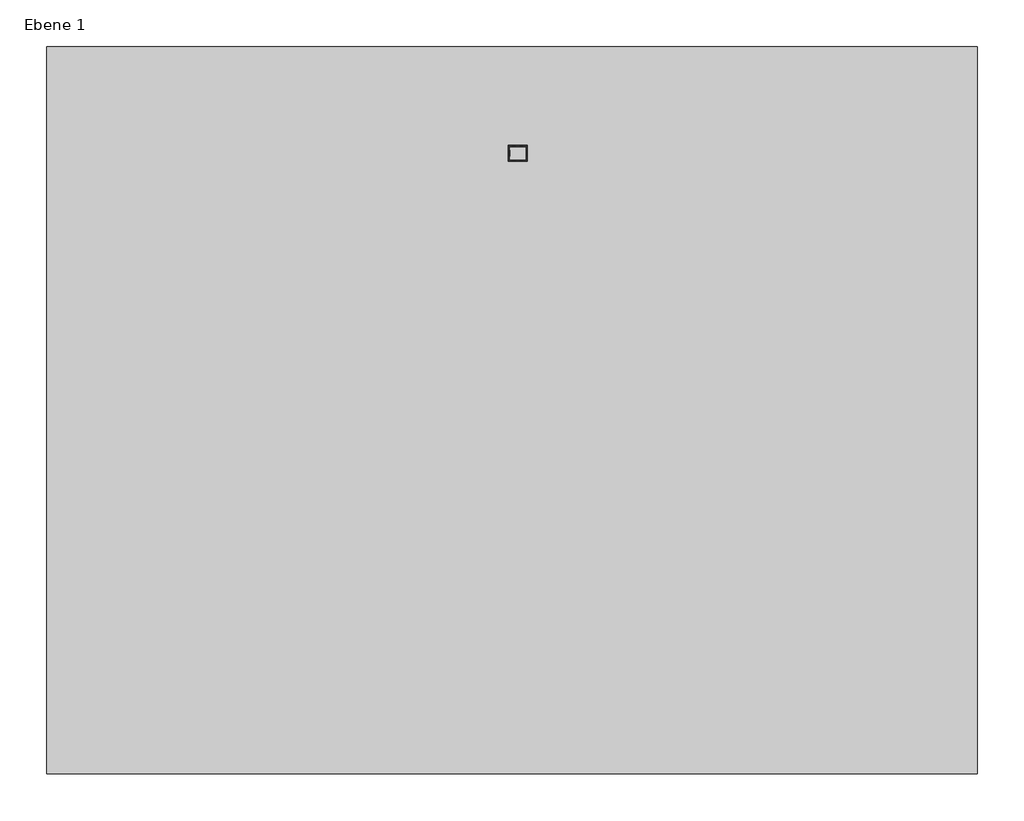
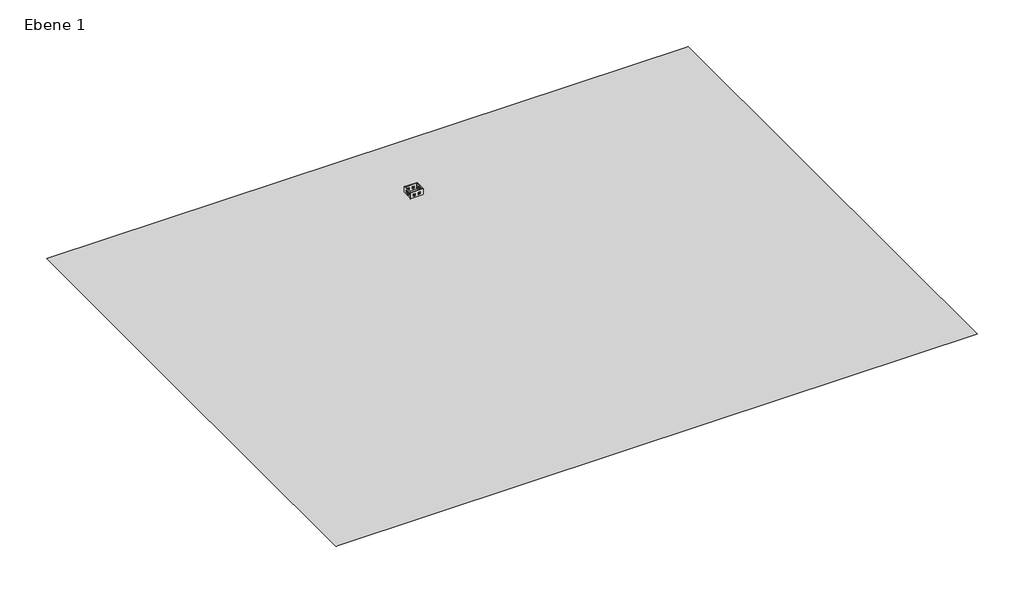
# One storey: 6 windows, 4 walls, 2 proxies.
"""IFC4 building model written with IfcOpenShell, lengths in millimetres."""

import ifcopenshell
import ifcopenshell.guid

model = None  # the IFC model being written
_history = None  # IfcOwnerHistory: only IFC2X3 demands one
_inside = {}  # id of a spatial element -> (the spatial element, [elements in it])
_under = {}  # id of a project, library or spatial element -> (it, [spatial elements below it])
_declared = {}  # id of a project -> (the project, [libraries it declares])
_typed = {}  # id of a type object -> (the type object, [elements of that type])
_made_of = {}  # id of a material, layer set ... -> (it, [elements and type objects made of it])


def new_model(schema):
    """Start an empty IFC model of exactly this schema.

    Asked for "IFC4X3", IfcOpenShell would pick the latest addendum, in which some entities
    have other attributes; the version numbers below select the first issue.
    IFC2X3 requires an IfcOwnerHistory on every rooted entity: one is made here for all.
    """
    global model, _history
    if schema == "IFC4X3":
        model = ifcopenshell.file(schema_version=(4, 3, 0, 0))
    else:
        model = ifcopenshell.file(schema=schema)
    _inside.clear()
    _under.clear()
    _declared.clear()
    _typed.clear()
    _made_of.clear()
    _history = None
    if model.schema == "IFC2X3":
        org = make("IfcOrganization", Name="unknown")
        user = make(
            "IfcPersonAndOrganization",
            ThePerson=make("IfcPerson", FamilyName="unknown"),
            TheOrganization=org,
        )
        app = make(
            "IfcApplication",
            ApplicationDeveloper=org,
            Version="unknown",
            ApplicationFullName="unknown",
            ApplicationIdentifier="unknown",
        )
        _history = make(
            "IfcOwnerHistory",
            OwningUser=user,
            OwningApplication=app,
            ChangeAction="ADDED",
            CreationDate=0,
        )
    return model


def make(cls, **values):
    """One entity of the class cls with the attributes given. An attribute that is None is left unset."""
    return model.create_entity(
        cls, **{name: value for name, value in values.items() if value is not None}
    )


def rooted(cls, **values):
    """An entity with a GlobalId (a new one), such as an element, a storey or a relation."""
    return make(cls, GlobalId=ifcopenshell.guid.new(), OwnerHistory=_history, **values)


def si_unit(unit_type, name, prefix=None):
    """IfcSIUnit, for example si_unit("LENGTHUNIT", "METRE", prefix="MILLI")."""
    return make("IfcSIUnit", UnitType=unit_type, Prefix=prefix, Name=name)


def assignment(units):
    """IfcUnitAssignment: the units of a project."""
    return None if units is None else make("IfcUnitAssignment", Units=units)


def point(xyz):
    """IfcCartesianPoint."""
    return None if xyz is None else make("IfcCartesianPoint", Coordinates=xyz)


def direction(xyz):
    """IfcDirection."""
    return None if xyz is None else make("IfcDirection", DirectionRatios=xyz)


def frame(location, z_axis=None, x_axis=None):
    """IfcAxis2Placement3D, a coordinate frame: its origin and axes. An axis left out is left unset."""
    return make(
        "IfcAxis2Placement3D",
        Location=point(location),
        Axis=direction(z_axis),
        RefDirection=direction(x_axis),
    )


def origin():
    """The frame at (0, 0, 0) with its axes left unset."""
    return frame((0.0, 0.0, 0.0))


def place(relative_to, where):
    """IfcLocalPlacement: puts the frame where relative to a parent placement (None: the world)."""
    return make(
        "IfcLocalPlacement", PlacementRelTo=relative_to, RelativePlacement=where
    )


def context(
    kind, dimensions, precision=None, world=None, true_north=None, identifier=None
):
    """IfcGeometricRepresentationContext, for example the 3D "Model" context."""
    return make(
        "IfcGeometricRepresentationContext",
        ContextIdentifier=identifier,
        ContextType=kind,
        CoordinateSpaceDimension=dimensions,
        Precision=precision,
        WorldCoordinateSystem=world,
        TrueNorth=true_north,
    )


def project(units=None, contexts=None):
    """IfcProject with its units and contexts."""
    return rooted(
        "IfcProject",
        Name="project",
        RepresentationContexts=contexts,
        UnitsInContext=assignment(units),
    )


def spatial(cls, under=None, at=None, **own):
    """A site, building, storey or space (cls), placed at a placement, below another one or the project."""
    s = rooted(cls, ObjectPlacement=at, **own)
    if under is not None:
        _under.setdefault(under.id(), (under, []))[1].append(s)
    return s


def polyline(points):
    """IfcPolyline through the points."""
    return make("IfcPolyline", Points=[point(p) for p in points])


def point_list(points):
    """IfcCartesianPointList2D or 3D."""
    cls = (
        "IfcCartesianPointList2D" if len(points[0]) == 2 else "IfcCartesianPointList3D"
    )
    return make(cls, CoordList=points)


def outline(outer, holes=None, kind="AREA"):
    """IfcArbitraryClosedProfileDef: a profile drawn as a closed curve; with holes, ...WithVoids."""
    if holes is None:
        return make("IfcArbitraryClosedProfileDef", ProfileType=kind, OuterCurve=outer)
    return make(
        "IfcArbitraryProfileDefWithVoids",
        ProfileType=kind,
        OuterCurve=outer,
        InnerCurves=holes,
    )


def extrude(swept, where, along, depth):
    """IfcExtrudedAreaSolid: the profile swept, set in the frame where, extruded along a direction by depth."""
    return make(
        "IfcExtrudedAreaSolid",
        SweptArea=swept,
        Position=where,
        ExtrudedDirection=direction(along),
        Depth=depth,
    )


def faces_of(points, faces, orient=None, outer=None):
    """IfcFace entities. A face is a list of loops; a loop is a list of indices into points, from 0.

    orient and outer hold one flag for each loop. By default every Orientation is true, the
    first loop of a face is its IfcFaceOuterBound and the others are IfcFaceBound.
    """
    made = []
    for i, loops in enumerate(faces):
        bounds = []
        for j, loop in enumerate(loops):
            is_outer = j == 0 if outer is None else outer[i][j]
            bounds.append(
                make(
                    "IfcFaceOuterBound" if is_outer else "IfcFaceBound",
                    Bound=make("IfcPolyLoop", Polygon=[points[k] for k in loop]),
                    Orientation=True if orient is None else orient[i][j],
                )
            )
        made.append(make("IfcFace", Bounds=bounds))
    return made


def faceted_brep(points, faces, orient=None, outer=None, voids=None):
    """IfcFacetedBrep: a solid bounded by flat faces; with voids (closed shells), ...WithVoids."""
    shared = [point(p) for p in points]
    hull = make("IfcClosedShell", CfsFaces=faces_of(shared, faces, orient, outer))
    if voids is None:
        return make("IfcFacetedBrep", Outer=hull)
    return make(
        "IfcFacetedBrepWithVoids",
        Outer=hull,
        Voids=[
            make(cls, CfsFaces=faces_of(shared, fs, o, b)) for cls, fs, o, b in voids
        ],
    )


def triangles(points, corners, closed=None, point_numbers=None):
    """IfcTriangulatedFaceSet: each triangle names its three corners, points numbered from 1."""
    return make(
        "IfcTriangulatedFaceSet",
        Coordinates=point_list(points),
        Closed=closed,
        CoordIndex=corners,
        PnIndex=point_numbers,
    )


def shape(context_of_items, identifier, shape_type, items):
    """IfcShapeRepresentation: the items that make up one representation, for example the "Body"."""
    return make(
        "IfcShapeRepresentation",
        ContextOfItems=context_of_items,
        RepresentationIdentifier=identifier,
        RepresentationType=shape_type,
        Items=items,
    )


def source(mapping_origin, context_of_items, identifier, shape_type, items):
    """IfcRepresentationMap: a shape defined once, which mapped items show again and again."""
    return make(
        "IfcRepresentationMap",
        MappingOrigin=mapping_origin,
        MappedRepresentation=shape(context_of_items, identifier, shape_type, items),
    )


def transform(
    local_origin,
    x_axis=None,
    y_axis=None,
    z_axis=None,
    scale=None,
    scale2=None,
    scale3=None,
    uniform=True,
):
    """IfcCartesianTransformationOperator3D, or its non-uniform kind. x_axis, y_axis, z_axis: its Axis1, 2, 3."""
    if uniform:
        return make(
            "IfcCartesianTransformationOperator3D",
            Axis1=direction(x_axis),
            Axis2=direction(y_axis),
            LocalOrigin=point(local_origin),
            Scale=scale,
            Axis3=direction(z_axis),
        )
    return make(
        "IfcCartesianTransformationOperator3DnonUniform",
        Axis1=direction(x_axis),
        Axis2=direction(y_axis),
        LocalOrigin=point(local_origin),
        Scale=scale,
        Axis3=direction(z_axis),
        Scale2=scale2,
        Scale3=scale3,
    )


def mapped(mapping_source, mapping_target):
    """IfcMappedItem: shows the shape of a source again, moved by a transform."""
    return make(
        "IfcMappedItem", MappingSource=mapping_source, MappingTarget=mapping_target
    )


def made_of(thing, what):
    """Note that an element or type object is made of a material, layer set ...; save() writes the relation."""
    if what is not None:
        _made_of.setdefault(what.id(), (what, []))[1].append(thing)
    return thing


def element(
    cls,
    number,
    at=None,
    inside=None,
    cuts=None,
    type_object=None,
    material=None,
    context=None,
    identifier="Body",
    shape_type=None,
    held_by="IfcProductDefinitionShape",
    body=None,
    shapes=None,
    **own,
):
    """One element of the class cls, such as IfcWall. Its Tag is "e" and its number.

    at: its placement. inside: the storey or other place that contains it. cuts: it is an
    opening in that element (IfcRelVoidsElement). A single representation is given by context,
    identifier, shape_type and body (its items); several are given by shapes. held_by: the class
    of the entity that holds the representations. save() writes the other relations.
    """
    e = rooted(cls, Tag="e%d" % number, ObjectPlacement=at, **own)
    if body is not None:
        shapes = [shape(context, identifier, shape_type, body)]
    if shapes is not None:
        e.Representation = make(held_by, Representations=shapes)
    if inside is not None:
        _inside.setdefault(inside.id(), (inside, []))[1].append(e)
    if cuts is not None:
        rooted(
            "IfcRelVoidsElement", RelatingBuildingElement=cuts, RelatedOpeningElement=e
        )
    if type_object is not None:
        _typed.setdefault(type_object.id(), (type_object, []))[1].append(e)
    return made_of(e, material)


def aggregate(whole, parts):
    """IfcRelAggregates: a whole, such as a stair, and the parts it consists of."""
    return rooted("IfcRelAggregates", RelatingObject=whole, RelatedObjects=parts)


def save(model, path):
    """Write the relations noted so far, then the file.

    IfcRelAggregates (storeys below a building ...), IfcRelContainedInSpatialStructure (elements
    in a storey), IfcRelDefinesByType, IfcRelAssociatesMaterial and IfcRelDeclares: one each for
    every whole, place, type object, material and project.
    """
    for whole, parts in _under.values():
        aggregate(whole, parts)
    for where, things in _inside.values():
        rooted(
            "IfcRelContainedInSpatialStructure",
            RelatedElements=things,
            RelatingStructure=where,
        )
    for kind, things in _typed.values():
        rooted("IfcRelDefinesByType", RelatedObjects=things, RelatingType=kind)
    for what, things in _made_of.values():
        rooted("IfcRelAssociatesMaterial", RelatedObjects=things, RelatingMaterial=what)
    for by, libraries in _declared.values():
        rooted("IfcRelDeclares", RelatingContext=by, RelatedDefinitions=libraries)
    model.write(path)


def fenster_1_flg_variabel_fenster_1_flg_variabel_3_8a378bad(model_context):
    return source(origin(), model_context, "Body", "SolidModel", [
        extrude(outline(polyline([(2010.0, 505.0), (2010.0, -505.0), (1000.0, -505.0), (1000.0, 505.0), (2010.0, 505.0)]), holes=[polyline([(1930.0, 445.0), (1080.0, 445.0), (1080.0, -445.0), (1930.0, -445.0), (1930.0, 445.0)])]), frame((0.0, 40.0, 0.0), z_axis=(0.0, 1.0, 0.0), x_axis=(0.0, 0.0, 1.0)), (0.0, 0.0, 1.0), 60.0),
        faceted_brep([(475.0, 40.0, 1960.0), (475.0, 10.0, 1960.0), (475.0, 10.0, 1050.0), (475.0, 40.0, 1050.0), (-475.0, 10.0, 1960.0), (-475.0, 10.0, 1050.0), (415.0, 10.0, 1110.0), (-415.0, 10.0, 1110.0), (-415.0, 10.0, 1900.0), (415.0, 10.0, 1900.0), (-475.0, 40.0, 1050.0), (-475.0, 40.0, 1960.0), (445.0, 40.0, 1930.0), (-445.0, 40.0, 1930.0), (-445.0, 40.0, 1080.0), (445.0, 40.0, 1080.0), (445.0, 70.0, 1930.0), (445.0, 70.0, 1080.0), (-445.0, 70.0, 1080.0), (-445.0, 70.0, 1930.0), (415.0, 70.0, 1900.0), (-415.0, 70.0, 1900.0), (-415.0, 70.0, 1110.0), (415.0, 70.0, 1110.0)], [[[0, 1, 2, 3]], [[1, 4, 5, 2], [6, 7, 8, 9]], [[3, 2, 5, 10]], [[3, 10, 11, 0], [12, 13, 14, 15]], [[16, 12, 15, 17]], [[17, 15, 14, 18]], [[17, 18, 19, 16], [20, 21, 22, 23]], [[9, 20, 23, 6]], [[6, 23, 22, 7]], [[10, 5, 4, 11]], [[18, 14, 13, 19]], [[7, 22, 21, 8]], [[11, 4, 1, 0]], [[19, 13, 12, 16]], [[8, 21, 20, 9]]]),
        extrude(outline(polyline([(-505.0, -210.0), (-505.0, 40.0), (505.0, 40.0), (505.0, -210.0), (-505.0, -210.0)])), frame((0.0, 0.0, 1005.0), z_axis=(0.0, 0.0, 1.0), x_axis=(1.0, 0.0, 0.0)), (0.0, 0.0, 1.0), 15.0),
        extrude(outline(polyline([(110.0221543, 1020.0), (210.0, 1000.0), (210.0, 990.0), (208.0, 990.0), (208.0, 998.3604634), (109.8240723, 1018.0), (100.0, 1018.0), (100.0, 1020.0), (110.0221543, 1020.0)])), frame((-505.0, 0.0, 0.0), z_axis=(1.0, 0.0, 0.0), x_axis=(0.0, 1.0, 0.0)), (0.0, 0.0, 1.0), 1010.0),
        extrude(outline(polyline([(415.0, 25.0), (-415.0, 25.0), (-415.0, 55.0), (415.0, 55.0), (415.0, 25.0)])), frame((0.0, 0.0, 1110.0), z_axis=(0.0, 0.0, 1.0), x_axis=(1.0, 0.0, 0.0)), (0.0, 0.0, 1.0), 790.0),
    ])


def fenster_2_flg_variabel_fenster_2_flg_variabel_3_03287464(model_context):
    return source(origin(), model_context, "Body", "SolidModel", [
        extrude(outline(polyline([(60.0, -5.0), (915.0, -5.0), (915.0, -35.0), (60.0, -35.0), (60.0, -5.0)])), frame((0.0, 0.0, 1110.0), z_axis=(0.0, 0.0, 1.0), x_axis=(1.0, 0.0, 0.0)), (0.0, 0.0, 1.0), 1040.0),
        extrude(outline(polyline([(-915.0, -5.0), (-60.0, -5.0), (-60.0, -35.0), (-915.0, -35.0), (-915.0, -5.0)])), frame((0.0, 0.0, 1110.0), z_axis=(0.0, 0.0, 1.0), x_axis=(1.0, 0.0, 0.0)), (0.0, 0.0, 1.0), 1040.0),
        extrude(outline(polyline([(-1005.0, -210.0), (-1005.0, -20.0), (1005.0, -20.0), (1005.0, -210.0), (-1005.0, -210.0)])), frame((0.0, 0.0, 1005.0), z_axis=(0.0, 0.0, 1.0), x_axis=(1.0, 0.0, 0.0)), (0.0, 0.0, 1.0), 15.0),
        extrude(outline(polyline([(50.0221543, 1020.0), (210.0, 1000.0), (210.0, 990.0), (208.0, 990.0), (208.0, 998.3604634), (49.8240723, 1018.0), (40.0, 1018.0), (40.0, 1020.0), (50.0221543, 1020.0)])), frame((-1005.0, 0.0, 0.0), z_axis=(1.0, 0.0, 0.0), x_axis=(0.0, 1.0, 0.0)), (0.0, 0.0, 1.0), 2010.0),
        extrude(outline(polyline([(30.0, -20.0), (-30.0, -20.0), (-30.0, 40.0), (30.0, 40.0), (30.0, -20.0)])), frame((0.0, 0.0, 1080.0), z_axis=(0.0, 0.0, 1.0), x_axis=(1.0, 0.0, 0.0)), (0.0, 0.0, 1.0), 1100.0),
        extrude(outline(polyline([(2260.0, -1005.0), (1000.0, -1005.0), (1000.0, 1005.0), (2260.0, 1005.0), (2260.0, -1005.0)]), holes=[polyline([(2180.0, -945.0), (2180.0, 945.0), (1080.0, 945.0), (1080.0, -945.0), (2180.0, -945.0)])]), frame((0.0, -20.0, 0.0), z_axis=(0.0, 1.0, 0.0), x_axis=(0.0, 0.0, 1.0)), (0.0, 0.0, 1.0), 60.0),
        faceted_brep([(-945.0, -20.0, 1080.0), (-945.0, 10.0, 1080.0), (-30.0, 10.0, 1080.0), (-30.0, -20.0, 1080.0), (-30.0, 10.0, 2180.0), (-30.0, -20.0, 2180.0), (-945.0, 10.0, 2180.0), (-60.0, 10.0, 2150.0), (-915.0, 10.0, 2150.0), (-915.0, 10.0, 1110.0), (-60.0, 10.0, 1110.0), (0.0, -20.0, 1050.0), (-975.0, -20.0, 1050.0), (-975.0, -20.0, 2210.0), (0.0, -20.0, 2210.0), (-945.0, -20.0, 2180.0), (-975.0, -50.0, 1050.0), (0.0, -50.0, 1050.0), (0.0, -50.0, 2210.0), (-975.0, -50.0, 2210.0), (-60.0, -50.0, 1110.0), (-915.0, -50.0, 1110.0), (-915.0, -50.0, 2150.0), (-60.0, -50.0, 2150.0)], [[[0, 1, 2, 3]], [[3, 2, 4, 5]], [[2, 1, 6, 4], [7, 8, 9, 10]], [[11, 12, 13, 14], [5, 15, 0, 3]], [[16, 12, 11, 17]], [[17, 11, 14, 18]], [[18, 19, 16, 17], [20, 21, 22, 23]], [[9, 21, 20, 10]], [[10, 20, 23, 7]], [[15, 6, 1, 0]], [[19, 13, 12, 16]], [[8, 22, 21, 9]], [[5, 4, 6, 15]], [[18, 14, 13, 19]], [[7, 23, 22, 8]]]),
        faceted_brep([(30.0, -20.0, 1080.0), (30.0, 10.0, 1080.0), (945.0, 10.0, 1080.0), (945.0, -20.0, 1080.0), (945.0, 10.0, 2180.0), (945.0, -20.0, 2180.0), (30.0, 10.0, 2180.0), (915.0, 10.0, 2150.0), (60.0, 10.0, 2150.0), (60.0, 10.0, 1110.0), (915.0, 10.0, 1110.0), (975.0, -20.0, 1050.0), (0.0, -20.0, 1050.0), (0.0, -20.0, 2210.0), (975.0, -20.0, 2210.0), (30.0, -20.0, 2180.0), (0.0, -50.0, 1050.0), (975.0, -50.0, 1050.0), (975.0, -50.0, 2210.0), (0.0, -50.0, 2210.0), (915.0, -50.0, 1110.0), (60.0, -50.0, 1110.0), (60.0, -50.0, 2150.0), (915.0, -50.0, 2150.0)], [[[0, 1, 2, 3]], [[3, 2, 4, 5]], [[2, 1, 6, 4], [7, 8, 9, 10]], [[11, 12, 13, 14], [5, 15, 0, 3]], [[16, 12, 11, 17]], [[17, 11, 14, 18]], [[18, 19, 16, 17], [20, 21, 22, 23]], [[9, 21, 20, 10]], [[10, 20, 23, 7]], [[15, 6, 1, 0]], [[19, 13, 12, 16]], [[8, 22, 21, 9]], [[5, 4, 6, 15]], [[18, 14, 13, 19]], [[7, 23, 22, 8]]]),
    ])


model = new_model("IFC4")

# Units and contexts
model_context = context("Model", 3, world=origin())
ifc_project = project(units=[si_unit("LENGTHUNIT", "METRE", prefix="MILLI")], contexts=[model_context])

# Site, building, storey
site = spatial("IfcSite", under=ifc_project)
building = spatial("IfcBuilding", under=site)
storey = spatial("IfcBuildingStorey", under=building, Name="Ebene 1", Elevation=3000.0)

# Proxies
placement = place(None, origin())
element("IfcBuildingElementProxy", 1, Name="Building Element Proxy", at=placement, inside=storey, context=model_context, shape_type="Tessellation", body=[
    triangles([(-160331.1996094, -65742.4011108, 3048.0), (-160331.1996094, -208151.4062988, 3048.0), (23848.9001038, -208151.4062988, 3048.0), (12197.4996643, -199419.9020508, 3048.0), (-5694.3001007, -186011.6041992, 3048.0), (-25481.9004272, -171004.4085938, 3048.0), (-41498.6018555, -156049.302832, 3048.0), (-55953.3009521, -142550.7035156, 3048.0), (-81517.601001, -122551.5986572, 3048.0), (-90344.9970703, -115644.9969727, 3048.0), (-95745.3, -111898.3977539, 3048.0), (-139582.1033203, -81515.7034424, 3048.0), (154493.6024414, -208151.4062988, 3048.0), (154493.6024414, -146509.2990967, 3048.0), (152327.2974609, -183778.6986328, 3048.0), (151970.2029785, -191029.9025391, 3048.0), (131234.6407471, -189976.3854492, 3048.0), (128010.9956543, -189812.6000977, 3048.0), (103567.5016113, -191451.7000488, 3048.0), (73532.4977051, -193637.296875, 3048.0), (59545.7979492, -197106.1083984, 3048.0), (45621.6990234, -200561.3021484, 3048.0), (35421.8006836, -204117.6060059, 3048.0), (25840.2994812, -207458.2951172, 3048.0), (154493.6024414, 37859.0007568, 3048.0), (-45179.0004639, 37859.0007568, 3048.0), (-20995.999823, -3482.9999016, 3048.0), (-20185.0004883, -4870.0001244, 3048.0), (-16502.099707, -11166.2998169, 3048.0), (-5863.3002502, -5298.2998535, 3048.0), (4055.6001251, 223.0999905, 3048.0), (14232.299881, 5042.7997513, 3048.0), (20896.8988953, 7816.7002029, 3048.0), (23379.4008545, 2726.9001228, 3048.0), (32183.900647, -15324.6994812, 3048.0), (35127.4000488, -15951.6995819, 3048.0), (51396.7000122, -19416.9996918, 3048.0), (71552.5022827, -34777.0005066, 3048.0), (89162.3994873, -48196.3000122, 3048.0), (97424.6021484, -54516.300293, 3048.0), (103453.3969482, -59668.902063, 3048.0), (125381.6956787, -79503.9006592, 3048.0), (138980.4005127, -76672.5013916, 3048.0), (142103.1959473, -85544.0994141, 3048.0), (152666.9046387, -116932.3044434, 3048.0), (-160331.1996094, 37859.0007568, 3048.0), (-157617.8024414, -59206.6000488, 3048.0), (-156348.2055176, -56148.4006714, 3048.0), (-133528.5007324, -3798.9000961, 3048.0), (-116015.0022949, -11087.9999451, 3048.0), (-107594.0000244, -6686.0000336, 3048.0), (-104346.1517578, -5888.8399704, 3048.0), (-103918.9964355, -5783.9998581, 3048.0), (-102571.999585, -5452.9997131, 3048.0), (-102346.0040771, -5318.9997528, 3048.0), (-100888.0000488, -4452.9999962, 3048.0), (-98390.0036865, -3171.9999893, 3048.0), (-95145.0017578, -1507.0000202, 3048.0), (-87760.0013672, 3877.9999191, 3048.0), (-87175.9998047, 4304.0000793, 3048.0), (-73718.9979492, 7734.0000183, 3048.0), (-75124.0005615, 10122.9995453, 3048.0), (-76451.9985718, 12378.0002747, 3048.0), (-73623.9990967, 14575.9998322, 3048.0), (-67567.0013672, 20473.9991272, 3048.0), (-64063.0012939, 24429.9995178, 3048.0), (-58507.0008911, 30701.0004639, 3048.0), (-58376.9995239, 30747.9999207, 3048.0)], [[1, 2, 12], [47, 12, 48], [12, 47, 1], [50, 12, 11], [46, 1, 47], [48, 50, 49], [48, 12, 50], [56, 51, 52], [52, 51, 50], [50, 53, 52], [50, 51, 49], [12, 2, 11], [46, 47, 48], [10, 29, 11], [9, 2, 8], [9, 29, 10], [8, 2, 7], [10, 2, 9], [9, 8, 29], [53, 54, 55], [53, 50, 54], [57, 55, 11], [11, 55, 54], [11, 2, 10], [58, 11, 29], [50, 11, 54], [52, 53, 56], [35, 8, 7], [7, 2, 6], [2, 5, 6], [55, 56, 53], [51, 57, 49], [57, 51, 56], [49, 57, 59], [57, 11, 58], [55, 57, 56], [59, 57, 58], [46, 59, 60], [59, 46, 49], [60, 63, 46], [63, 60, 62], [59, 61, 60], [46, 63, 65], [58, 61, 59], [49, 46, 48], [62, 61, 64], [61, 62, 60], [65, 61, 27], [61, 65, 64], [27, 61, 28], [62, 64, 63], [66, 46, 65], [65, 27, 66], [67, 68, 26], [68, 67, 66], [68, 66, 27], [67, 26, 46], [26, 68, 27], [67, 46, 66], [27, 31, 26], [63, 64, 65], [58, 29, 61], [7, 6, 38], [4, 3, 24], [24, 13, 23], [4, 24, 23], [21, 22, 23], [21, 23, 13], [4, 23, 22], [4, 22, 5], [4, 5, 2], [5, 21, 39], [13, 20, 21], [22, 21, 5], [20, 40, 21], [24, 3, 13], [3, 4, 2], [18, 13, 17], [13, 18, 19], [16, 13, 15], [13, 16, 17], [19, 20, 13], [17, 16, 15], [19, 18, 14], [42, 19, 45], [45, 19, 14], [14, 15, 13], [45, 14, 25], [18, 17, 14], [17, 15, 14], [44, 45, 25], [19, 42, 20], [44, 42, 45], [28, 29, 30], [28, 61, 29], [30, 35, 31], [35, 30, 29], [35, 29, 8], [30, 31, 27], [32, 26, 31], [32, 31, 34], [37, 33, 34], [34, 33, 32], [31, 35, 34], [33, 26, 32], [34, 35, 36], [28, 30, 27], [25, 40, 41], [39, 38, 6], [42, 43, 41], [43, 42, 44], [40, 39, 21], [25, 41, 43], [37, 25, 33], [37, 36, 38], [38, 39, 25], [36, 35, 7], [25, 39, 40], [38, 25, 37], [38, 36, 7], [37, 34, 36], [43, 44, 25], [41, 40, 20], [20, 42, 41], [33, 25, 26], [39, 6, 5]], closed=False),
])
element("IfcBuildingElementProxy", 2, Name="Building Element Proxy", at=placement, inside=storey, context=model_context, shape_type="Tessellation", body=[
    triangles([(-20995.999823, -3482.9999016, 3048.0), (-45179.0004639, 37859.0007568, 3048.0), (-58376.9995239, 30747.9999207, 3048.0), (-58507.0008911, 30701.0004639, 3048.0), (-64063.0012939, 24429.9995178, 3048.0), (-67567.0013672, 20473.9991272, 3048.0), (-73623.9990967, 14575.9998322, 3048.0), (-76451.9985718, 12378.0002747, 3048.0), (-75124.0005615, 10122.9995453, 3048.0), (-73718.9979492, 7734.0000183, 3048.0), (-87175.9998047, 4304.0000793, 3048.0), (-87760.0013672, 3877.9999191, 3048.0), (-95145.0017578, -1507.0000202, 3048.0), (-98390.0036865, -3171.9999893, 3048.0), (-100888.0000488, -4452.9999962, 3048.0), (-102346.0040771, -5318.9997528, 3048.0), (-102571.999585, -5452.9997131, 3048.0), (-103918.9964355, -5783.9998581, 3048.0), (-104346.1517578, -5888.8399704, 3048.0), (-107594.0000244, -6686.0000336, 3048.0), (-116015.0022949, -11087.9999451, 3048.0), (-133528.5007324, -3798.9000961, 3048.0), (-156348.2055176, -56148.4006714, 3048.0), (-157617.8024414, -59206.6000488, 3048.0), (-160331.1996094, -65742.4011108, 3048.0), (-139582.1033203, -81515.7034424, 3048.0), (-95745.3, -111898.3977539, 3048.0), (-90344.9970703, -115644.9969727, 3048.0), (-81517.601001, -122551.5986572, 3048.0), (-55953.3009521, -142550.7035156, 3048.0), (-41498.6018555, -156049.302832, 3048.0), (-25481.9004272, -171004.4085938, 3048.0), (-5694.3001007, -186011.6041992, 3048.0), (12197.4996643, -199419.9020508, 3048.0), (23848.9001038, -208151.4062988, 3048.0), (25840.2994812, -207458.2951172, 3048.0), (35421.8006836, -204117.6060059, 3048.0), (45621.6990234, -200561.3021484, 3048.0), (59545.7979492, -197106.1083984, 3048.0), (73532.4977051, -193637.296875, 3048.0), (103567.5016113, -191451.7000488, 3048.0), (128010.9956543, -189812.6000977, 3048.0), (131234.6407471, -189976.3854492, 3048.0), (151970.2029785, -191029.9025391, 3048.0), (152327.2974609, -183778.6986328, 3048.0), (154493.6024414, -146509.2990967, 3048.0), (152666.9046387, -116932.3044434, 3048.0), (142103.1959473, -85544.0994141, 3048.0), (138980.4005127, -76672.5013916, 3048.0), (125381.6956787, -79503.9006592, 3048.0), (103453.3969482, -59668.902063, 3048.0), (97424.6021484, -54516.300293, 3048.0), (89162.3994873, -48196.3000122, 3048.0), (71552.5022827, -34777.0005066, 3048.0), (51396.7000122, -19416.9996918, 3048.0), (35127.4000488, -15951.6995819, 3048.0), (32183.900647, -15324.6994812, 3048.0), (23379.4008545, 2726.9001228, 3048.0), (20896.8988953, 7816.7002029, 3048.0), (14232.299881, 5042.7997513, 3048.0), (4055.6001251, 223.0999905, 3048.0), (-5863.3002502, -5298.2998535, 3048.0), (-16502.099707, -11166.2998169, 3048.0), (-20185.0004883, -4870.0001244, 3048.0)], [[24, 25, 26], [23, 26, 21], [26, 23, 24], [20, 21, 19], [18, 19, 21], [18, 21, 17], [21, 26, 27], [23, 21, 22], [28, 63, 27], [29, 63, 28], [29, 30, 63], [16, 17, 27], [16, 27, 14], [17, 21, 27], [13, 27, 63], [57, 30, 31], [14, 27, 13], [16, 14, 15], [8, 9, 7], [10, 11, 12], [12, 13, 10], [10, 7, 9], [7, 10, 6], [6, 1, 5], [1, 6, 10], [1, 10, 64], [4, 5, 3], [3, 5, 1], [1, 2, 3], [13, 63, 10], [31, 32, 54], [34, 35, 36], [34, 36, 37], [34, 37, 38], [34, 38, 33], [33, 39, 53], [38, 39, 33], [40, 52, 39], [41, 42, 46], [42, 43, 46], [45, 43, 44], [46, 47, 41], [46, 43, 45], [41, 47, 50], [41, 50, 40], [48, 50, 47], [64, 10, 63], [62, 57, 61], [57, 62, 63], [57, 63, 30], [60, 61, 58], [58, 59, 60], [61, 57, 58], [53, 54, 32], [49, 50, 48], [52, 53, 39], [55, 56, 54], [56, 57, 31], [54, 56, 31], [51, 52, 40], [40, 50, 51], [53, 32, 33]], closed=False),
])

# Walls
element("IfcWall", 3, ObjectType="MW 24.0 WD 12.0", at=placement, inside=storey, context=model_context, shape_type="Brep", body=[
    faceted_brep([(-3766.4979049, 4044.3692517, 3000.0), (1873.5020951, 4044.3692517, 3000.0), (1873.5020951, 4044.3692517, 6000.0), (-3766.4979049, 4044.3692517, 6000.0), (673.5020951, 4044.3692517, 4000.0), (-336.4979049, 4044.3692517, 4000.0), (-336.4979049, 4044.3692517, 5010.0), (673.5020951, 4044.3692517, 5010.0), (-1756.4979049, 4044.3692517, 4000.0), (-2766.4979049, 4044.3692517, 4000.0), (-2766.4979049, 4044.3692517, 5010.0), (-1756.4979049, 4044.3692517, 5010.0), (-4126.4979049, 4404.3692517, 3000.0), (-4126.4979049, 4404.3692517, 6000.0), (2233.5020951, 4404.3692517, 6000.0), (2233.5020951, 4404.3692517, 3000.0), (673.5020951, 4404.3692517, 4000.0), (673.5020951, 4404.3692517, 5010.0), (-336.4979049, 4404.3692517, 5010.0), (-336.4979049, 4404.3692517, 4000.0), (-1756.4979049, 4404.3692517, 4000.0), (-1756.4979049, 4404.3692517, 5010.0), (-2766.4979049, 4404.3692517, 5010.0), (-2766.4979049, 4404.3692517, 4000.0)], [[[0, 1, 2, 3], [4, 5, 6, 7], [8, 9, 10, 11]], [[12, 13, 14, 15], [16, 17, 18, 19], [20, 21, 22, 23]], [[1, 0, 12, 15]], [[3, 2, 14, 13]], [[2, 1, 15, 14]], [[0, 3, 13, 12]], [[17, 16, 4, 7]], [[18, 17, 7, 6]], [[19, 18, 6, 5]], [[16, 19, 5, 4]], [[21, 20, 8, 11]], [[22, 21, 11, 10]], [[23, 22, 10, 9]], [[20, 23, 9, 8]]]),
])
element("IfcWall", 4, ObjectType="MW 24.0 WD 12.0", at=placement, inside=storey, context=model_context, shape_type="Brep", body=[
    faceted_brep([(1873.5020951, 4044.3692517, 3000.0), (1873.5020951, -595.6307483, 3000.0), (1873.5020951, -595.6307483, 6000.0), (1873.5020951, 4044.3692517, 6000.0), (1873.5020951, 719.3692517, 4000.0), (1873.5020951, 2729.3692517, 4000.0), (1873.5020951, 2729.3692517, 5260.0), (1873.5020951, 719.3692517, 5260.0), (2233.5020951, 4404.3692517, 3000.0), (2233.5020951, 4404.3692517, 6000.0), (2233.5020951, -955.6307483, 6000.0), (2233.5020951, -955.6307483, 3000.0), (2233.5020951, 719.3692517, 4000.0), (2233.5020951, 719.3692517, 5260.0), (2233.5020951, 2729.3692517, 5260.0), (2233.5020951, 2729.3692517, 4000.0)], [[[0, 1, 2, 3], [4, 5, 6, 7]], [[8, 9, 10, 11], [12, 13, 14, 15]], [[1, 0, 8, 11]], [[3, 2, 10, 9]], [[0, 3, 9, 8]], [[2, 1, 11, 10]], [[13, 12, 4, 7]], [[14, 13, 7, 6]], [[15, 14, 6, 5]], [[12, 15, 5, 4]]]),
])
element("IfcWall", 5, ObjectType="MW 24.0 WD 12.0", at=placement, inside=storey, context=model_context, shape_type="Brep", body=[
    faceted_brep([(1873.5020951, -595.6307483, 3000.0), (-3766.4979049, -595.6307483, 3000.0), (-3766.4979049, -595.6307483, 6000.0), (1873.5020951, -595.6307483, 6000.0), (-336.4979049, -595.6307483, 4000.0), (673.5020951, -595.6307483, 4000.0), (673.5020951, -595.6307483, 5010.0), (-336.4979049, -595.6307483, 5010.0), (-2766.4979049, -595.6307483, 4000.0), (-1756.4979049, -595.6307483, 4000.0), (-1756.4979049, -595.6307483, 5010.0), (-2766.4979049, -595.6307483, 5010.0), (2233.5020951, -955.6307483, 3000.0), (2233.5020951, -955.6307483, 6000.0), (-4126.4979049, -955.6307483, 6000.0), (-4126.4979049, -955.6307483, 3000.0), (-336.4979049, -955.6307483, 4000.0), (-336.4979049, -955.6307483, 5010.0), (673.5020951, -955.6307483, 5010.0), (673.5020951, -955.6307483, 4000.0), (-2766.4979049, -955.6307483, 4000.0), (-2766.4979049, -955.6307483, 5010.0), (-1756.4979049, -955.6307483, 5010.0), (-1756.4979049, -955.6307483, 4000.0)], [[[0, 1, 2, 3], [4, 5, 6, 7], [8, 9, 10, 11]], [[12, 13, 14, 15], [16, 17, 18, 19], [20, 21, 22, 23]], [[1, 0, 12, 15]], [[3, 2, 14, 13]], [[0, 3, 13, 12]], [[2, 1, 15, 14]], [[17, 16, 4, 7]], [[18, 17, 7, 6]], [[19, 18, 6, 5]], [[16, 19, 5, 4]], [[21, 20, 8, 11]], [[22, 21, 11, 10]], [[23, 22, 10, 9]], [[20, 23, 9, 8]]]),
])
element("IfcWall", 6, ObjectType="MW 24.0 WD 12.0", at=placement, inside=storey, context=model_context, shape_type="Brep", body=[
    faceted_brep([(-3766.4979049, -595.6307483, 3000.0), (-3766.4979049, 4044.3692517, 3000.0), (-3766.4979049, 4044.3692517, 6000.0), (-3766.4979049, -595.6307483, 6000.0), (-3766.4979049, 2729.3692517, 4000.0), (-3766.4979049, 719.3692517, 4000.0), (-3766.4979049, 719.3692517, 5260.0), (-3766.4979049, 2729.3692517, 5260.0), (-4126.4979049, -955.6307483, 3000.0), (-4126.4979049, -955.6307483, 6000.0), (-4126.4979049, 4404.3692517, 6000.0), (-4126.4979049, 4404.3692517, 3000.0), (-4126.4979049, 2729.3692517, 4000.0), (-4126.4979049, 2729.3692517, 5260.0), (-4126.4979049, 719.3692517, 5260.0), (-4126.4979049, 719.3692517, 4000.0)], [[[0, 1, 2, 3], [4, 5, 6, 7]], [[8, 9, 10, 11], [12, 13, 14, 15]], [[1, 0, 8, 11]], [[3, 2, 10, 9]], [[2, 1, 11, 10]], [[0, 3, 9, 8]], [[13, 12, 4, 7]], [[14, 13, 7, 6]], [[15, 14, 6, 5]], [[12, 15, 5, 4]]]),
])

# Windows
fenster_1_flg_variabel_fenster_1_flg_variabel_3_shape = fenster_1_flg_variabel_fenster_1_flg_variabel_3_8a378bad(model_context)
element("IfcWindow", 7, ObjectType="Fenster 1-flg - Variabel : Fenster 1-flg - Variabel 3", at=placement, inside=storey, context=model_context, shape_type="MappedRepresentation", body=[
    mapped(fenster_1_flg_variabel_fenster_1_flg_variabel_3_shape, transform((168.5020951, -775.6307483, 3000.0), x_axis=(1.0, 0.0, 0.0), y_axis=(0.0, 1.0, 0.0), z_axis=(0.0, 0.0, 1.0))),
])
element("IfcWindow", 8, ObjectType="Fenster 1-flg - Variabel : Fenster 1-flg - Variabel 3", at=placement, inside=storey, context=model_context, shape_type="MappedRepresentation", body=[
    mapped(fenster_1_flg_variabel_fenster_1_flg_variabel_3_shape, transform((-2261.4979049, -775.6307483, 3000.0), x_axis=(1.0, 0.0, 0.0), y_axis=(0.0, 1.0, 0.0), z_axis=(0.0, 0.0, 1.0))),
])
element("IfcWindow", 9, ObjectType="Fenster 1-flg - Variabel : Fenster 1-flg - Variabel 3", at=placement, inside=storey, context=model_context, shape_type="MappedRepresentation", body=[
    mapped(fenster_1_flg_variabel_fenster_1_flg_variabel_3_shape, transform((168.5020951, 4224.3692517, 3000.0), x_axis=(-1.0, 0.0, 0.0), y_axis=(0.0, -1.0, 0.0), z_axis=(0.0, 0.0, 1.0))),
])
element("IfcWindow", 10, ObjectType="Fenster 1-flg - Variabel : Fenster 1-flg - Variabel 3", at=placement, inside=storey, context=model_context, shape_type="MappedRepresentation", body=[
    mapped(fenster_1_flg_variabel_fenster_1_flg_variabel_3_shape, transform((-2261.4979049, 4224.3692517, 3000.0), x_axis=(-1.0, 0.0, 0.0), y_axis=(0.0, -1.0, 0.0), z_axis=(0.0, 0.0, 1.0))),
])
fenster_2_flg_variabel_fenster_2_flg_variabel_3_shape = fenster_2_flg_variabel_fenster_2_flg_variabel_3_03287464(model_context)
element("IfcWindow", 11, ObjectType="Fenster 2-flg - Variabel : Fenster 2-flg - Variabel 3", at=placement, inside=storey, context=model_context, shape_type="MappedRepresentation", body=[
    mapped(fenster_2_flg_variabel_fenster_2_flg_variabel_3_shape, transform((2053.5020951, 1724.3692517, 3000.0), x_axis=(0.0, 1.0, 0.0), y_axis=(-1.0, 0.0, 0.0), z_axis=(0.0, 0.0, 1.0))),
])
element("IfcWindow", 12, ObjectType="Fenster 2-flg - Variabel : Fenster 2-flg - Variabel 3", at=placement, inside=storey, context=model_context, shape_type="MappedRepresentation", body=[
    mapped(fenster_2_flg_variabel_fenster_2_flg_variabel_3_shape, transform((-3946.4979049, 1724.3692517, 3000.0), x_axis=(0.0, -1.0, 0.0), y_axis=(1.0, 0.0, 0.0), z_axis=(0.0, 0.0, 1.0))),
])

save(model, "model.ifc")

# Revit data of these elements
# Type "MW 24.0 WD 12.0"
#   Type Comments = "Mehrschaliges Mauerwerk"
#   Description = "Mauerwerk 24.0 cm, Wärmedämmung 12.0 cm"
#   Layers, outside or top first: 0.120 m "Wärmedämmung - hart" (function 3); 0.240 m "Mauerwerk - Ziegel, verputzt" (function 1)
# Type "Fenster 1-flg - Variabel : Fenster 1-flg - Variabel 3"
#   Type Mark = "52"
#   Operation = "SinglePanel"
#   Construction Type Id = "GSP4R"
#   Keynote = "16.05.01"
#   Analytic Construction = "1/8 Zoll Pilkington-Verglasung einfach"
#   Cost = 78.2
#   Visual Light Transmittance = 0.9
#   Höhe oberer  Rahmen = 0.080 m
#   Solar Heat Gain Coefficient = 0.86
#   Tiefe Flügel = 0.060 m
#   Rough Width [instance default] = 1.010 m
#   Rough Height [instance default] = 1.010 m
#   Rahmenhöhe unten = 0.080 m
#   Heat Transfer Coefficient (U) = 6.7069 W/(m²·K)
#   Rahmentiefe = 0.060 m
#   Rahmenbreite = 0.060 m
#   Height [instance default] = 1.010 m
#   Flügelbreite = 0.060 m
#   Einbautiefe (von außen) [instance default] = 0.080 m
#   Width [instance default] = 1.010 m
#   Define Thermal Properties by = 1
#   Öffnungsrichtung oben [instance default] = yes
#   Öffnungsrichtung in Draufsicht anzeigen [instance default] = no
#   Klappflügel [instance default] = no
#   Drehflügel 1 [instance default] = yes
#   Fensterflügel [instance default] = none
#   Innere Fensterbank [instance default] = none
#   Glas [instance default] = none
#   Bild [instance default] = none
#   Äußere Fensterbank [instance default] = none
#   Wall Closure = (empty or 0)
# Type "Fenster 2-flg - Variabel : Fenster 2-flg - Variabel 3"
#   Type Mark = "53"
#   Operation = "DoublePanelVertical"
#   Construction Type Id = "GSP4R"
#   Keynote = "16.05.01"
#   Analytic Construction = "1/8 Zoll Pilkington-Verglasung einfach"
#   Cost = 130.98
#   Visual Light Transmittance = 0.9
#   Solar Heat Gain Coefficient = 0.78
#   Rough Width [instance default] = 2.010 m
#   Rough Height [instance default] = 1.260 m
#   Heat Transfer Coefficient (U) = 3.6886 W/(m²·K)
#   Rahmentiefe = 0.060 m
#   Rahmenhöhe unten = 0.080 m
#   Höhe oberer  Rahmen = 0.080 m
#   Rahmenbreite = 0.060 m
#   Height [instance default] = 1.260 m
#   Tiefe Flügel = 0.060 m
#   Flügelbreite = 0.060 m
#   Einbautiefe (von außen) [instance default] = 0.140 m
#   Width [instance default] = 2.010 m
#   Define Thermal Properties by = 1
#   Öffnungsrichtung oben [instance default] = yes
#   Öffnungsrichtung in Draufsicht anzeigen [instance default] = no
#   Drehflügel 1 [instance default] = yes
#   Bild [instance default] = none
#   Glas [instance default] = none
#   Fensterflügel [instance default] = none
#   Äußere Fensterbank [instance default] = none
#   Innere Fensterbank [instance default] = none
#   Wall Closure = (empty or 0)
# Element 1 (IfcBuildingElementProxy)
#   Comments = "Reference plane: BP_Bereich"
#   Material = transparent
#   Phase Created = Phase 1
# Element 2 (IfcBuildingElementProxy)
#   Comments = "BP_Bereich"
#   boundedBy = "-"
#   nummer = "0"
#   geltungsbereich = "580779.815 5927135.13 580779.004 5927136.517 580754.821 5927177.859 580741.623 5927170.748 580741.493 5927170.701 580735.937 5927164.43 580732.433 5927160.474 580726.376 5927154.576 580723.548 5927152.378 580724.876 5927150.123 580726.281 5927147.734 580712.824 5927144.304 580712.24 5927143.878 580704.855 5927138.493 580701.61 5927136.828 580699.112 5927135.547 580697.654 5927134.681 580697.428 5927134.547 580696.081 5927134.216 580692.406 5927133.314 580683.985 5927128.912 580666.4715 5927136.2011 580643.6518 5927083.8516 580642.3822 5927080.7934 580639.6688 5927074.2576 580660.4179 5927058.4843 580704.2547 5927028.1016 580709.655 5927024.355 580718.4824 5927017.4484 580744.0467 5926997.4493 580758.5014 5926983.9507 580774.5181 5926968.9956 580794.3057 5926953.9884 580812.1975 5926940.5801 580823.8489 5926931.8486 580825.8403 5926932.5417 580835.4218 5926935.8824 580845.6217 5926939.4387 580859.5458 5926942.8939 580873.5325 5926946.3627 580903.5675 5926948.5483 580928.011 5926950.1874 580951.9702 5926948.9701 580952.3273 5926956.2213 580954.4936 5926993.4907 580952.6669 5927023.0677 580942.1032 5927054.4559 580938.9804 5927063.3275 580925.3817 5927060.4961 580903.4534 5927080.3311 580897.4246 5927085.4837 580889.1624 5927091.8037 580871.5525 5927105.223 580851.3967 5927120.583 580835.1274 5927124.0483 580832.1839 5927124.6753 580823.3794 5927142.7269 580820.8969 5927147.8167 580814.2323 5927145.0428 580804.0556 5927140.2231 580794.1367 5927134.7017 580783.4979 5927128.8337 580779.815 5927135.13"
#   refScan = "Bergedorf84.pgwBergedorf84.png"
#   planinhalt = ""
#   gehoertZuPlan = ""
#   Material = bereich
#   Phase Created = Phase 1
# Elements 3, 4, 5, 6 (IfcWall, "MW 24.0 WD 12.0")
#   Comments = ""
#   Top Offset = 0.000 m
#   Base Offset = 0.000 m
#   Unconnected Height = 3.000 m
#   wall height = 3.000 m
#   Phase Created = Phase 1
#   Base Constraint = Ebene 1
#   Materials on its faces: "Vorgabe - Wand", "Mauerwerk - Ziegel, verputzt", "Wärmedämmung - hart"
# Element 7 (IfcWindow, "Fenster 1-flg - Variabel : Fenster 1-flg - Variabel 3")
#   Mark = "2"
#   Rough Height = 1.010 m
#   Rough Width = 1.010 m
#   Height = 1.010 m
#   Einbautiefe (von außen) = 0.080 m
#   Width = 1.010 m
#   Öffnungsrichtung oben = yes
#   Öffnungsrichtung in Draufsicht anzeigen = no
#   Klappflügel = no
#   Drehflügel 1 = yes
#   Äußere Fensterbank = none
#   Innere Fensterbank = none
#   Glas = none
#   Fensterflügel = none
#   Bild = none
#   Phase Created = Phase 1
#   Materials on its faces: "Kunststoff - Weiß", "Holz - Birke", "Glas"
# Element 8 (IfcWindow, "Fenster 1-flg - Variabel : Fenster 1-flg - Variabel 3")
#   Mark = "3"
#   Rough Height = 1.010 m
#   Rough Width = 1.010 m
#   Height = 1.010 m
#   Einbautiefe (von außen) = 0.080 m
#   Width = 1.010 m
#   Öffnungsrichtung oben = yes
#   Öffnungsrichtung in Draufsicht anzeigen = no
#   Klappflügel = no
#   Drehflügel 1 = yes
#   Äußere Fensterbank = none
#   Innere Fensterbank = none
#   Glas = none
#   Fensterflügel = none
#   Bild = none
#   Phase Created = Phase 1
#   Materials on its faces: "Kunststoff - Weiß", "Holz - Birke", "Glas"
# Element 9 (IfcWindow, "Fenster 1-flg - Variabel : Fenster 1-flg - Variabel 3")
#   Mark = "4"
#   Rough Height = 1.010 m
#   Rough Width = 1.010 m
#   Height = 1.010 m
#   Einbautiefe (von außen) = 0.080 m
#   Width = 1.010 m
#   Öffnungsrichtung oben = yes
#   Öffnungsrichtung in Draufsicht anzeigen = no
#   Klappflügel = no
#   Drehflügel 1 = yes
#   Äußere Fensterbank = none
#   Innere Fensterbank = none
#   Glas = none
#   Fensterflügel = none
#   Bild = none
#   Phase Created = Phase 1
#   Materials on its faces: "Kunststoff - Weiß", "Holz - Birke", "Glas"
# Element 10 (IfcWindow, "Fenster 1-flg - Variabel : Fenster 1-flg - Variabel 3")
#   Mark = "5"
#   Rough Height = 1.010 m
#   Rough Width = 1.010 m
#   Height = 1.010 m
#   Einbautiefe (von außen) = 0.080 m
#   Width = 1.010 m
#   Öffnungsrichtung oben = yes
#   Öffnungsrichtung in Draufsicht anzeigen = no
#   Klappflügel = no
#   Drehflügel 1 = yes
#   Äußere Fensterbank = none
#   Innere Fensterbank = none
#   Glas = none
#   Fensterflügel = none
#   Bild = none
#   Phase Created = Phase 1
#   Materials on its faces: "Kunststoff - Weiß", "Holz - Birke", "Glas"
# Element 11 (IfcWindow, "Fenster 2-flg - Variabel : Fenster 2-flg - Variabel 3")
#   Mark = "8"
#   Rough Height = 1.260 m
#   Rough Width = 2.010 m
#   Height = 1.260 m
#   Einbautiefe (von außen) = 0.140 m
#   Width = 2.010 m
#   Öffnungsrichtung oben = yes
#   Öffnungsrichtung in Draufsicht anzeigen = no
#   Drehflügel 1 = yes
#   Äußere Fensterbank = none
#   Innere Fensterbank = none
#   Glas = none
#   Fensterflügel = none
#   Bild = none
#   Phase Created = Phase 1
#   Materials on its faces: "Kunststoff - Weiß", "Glas", "Holz - Birke"
# Element 12 (IfcWindow, "Fenster 2-flg - Variabel : Fenster 2-flg - Variabel 3")
#   Mark = "9"
#   Rough Height = 1.260 m
#   Rough Width = 2.010 m
#   Height = 1.260 m
#   Einbautiefe (von außen) = 0.140 m
#   Width = 2.010 m
#   Öffnungsrichtung oben = yes
#   Öffnungsrichtung in Draufsicht anzeigen = no
#   Drehflügel 1 = yes
#   Äußere Fensterbank = none
#   Innere Fensterbank = none
#   Glas = none
#   Fensterflügel = none
#   Bild = none
#   Phase Created = Phase 1
#   Materials on its faces: "Kunststoff - Weiß", "Glas", "Holz - Birke"
# Materials
#   "Wärmedämmung - hart": class "Stuck", colour RGB 255 255 255, transparency 0, Description = "Äußere Oberfläche", Cost = 0
#   "Mauerwerk - Ziegel, verputzt": class "Stuck", colour RGB 247 247 247, transparency 0, Cost = 0
#   "transparent": class "Nicht zugewiesen", colour RGB 0 0 0, transparency 1
#   "bereich": class "Nicht zugewiesen", colour RGB 0 0 0, transparency 1
#   "Vorgabe - Wand": class "Stuck", colour RGB 128 128 128, transparency 0, Description = "Äußere Oberfläche", Cost = 0
#   "Kunststoff - Weiß": class "Kunststoff", colour RGB 249 249 249, transparency 0, Cost = 0
#   "Holz - Birke": class "Holz", colour RGB 213 164 103, transparency 0, Cost = 0
#   "Glas": class "Glas", colour RGB 0 0 255, transparency 0.75, Comments = "Render-Darstellung nicht aktualisiert ", Cost = 0
